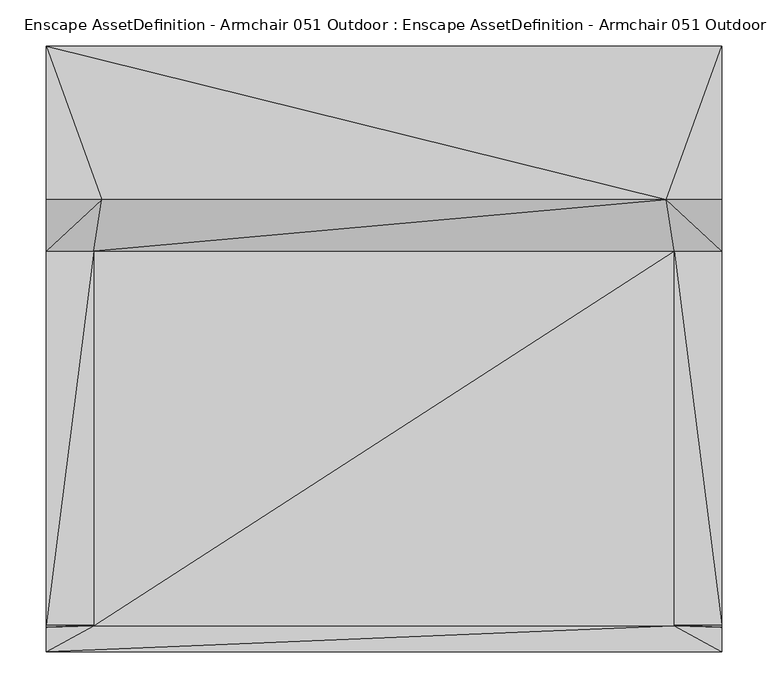
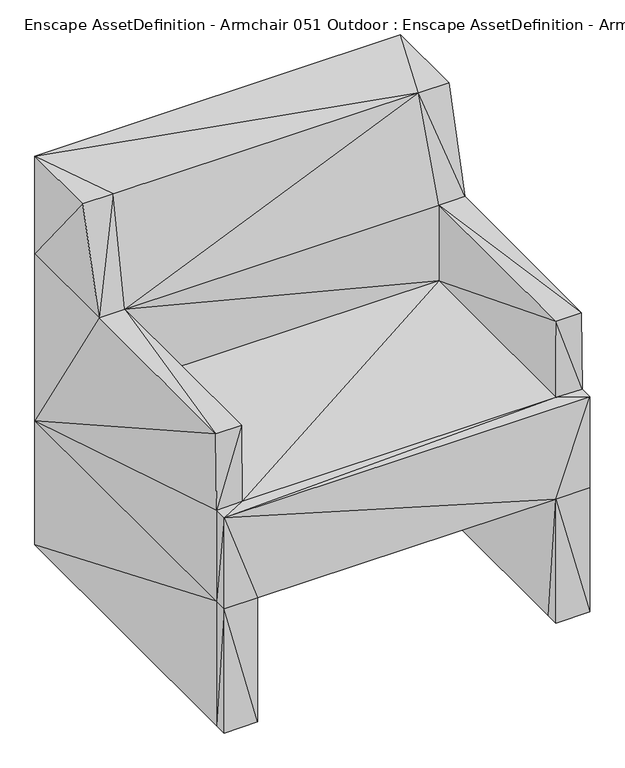
"""IFC4 building model written with IfcOpenShell, lengths in millimetres: geographic element geometry, Enscape AssetDefinition - Armchair 051 Outdoor : Enscape AssetDefinition - Armchair 051 Outdoor."""

import ifcopenshell
import ifcopenshell.guid

model = None  # the IFC model being written
_history = None  # IfcOwnerHistory: only IFC2X3 demands one
_inside = {}  # id of a spatial element -> (the spatial element, [elements in it])
_under = {}  # id of a project, library or spatial element -> (it, [spatial elements below it])
_declared = {}  # id of a project -> (the project, [libraries it declares])
_typed = {}  # id of a type object -> (the type object, [elements of that type])
_made_of = {}  # id of a material, layer set ... -> (it, [elements and type objects made of it])


def new_model(schema):
    """Start an empty IFC model of exactly this schema.

    Asked for "IFC4X3", IfcOpenShell would pick the latest addendum, in which some entities
    have other attributes; the version numbers below select the first issue.
    IFC2X3 requires an IfcOwnerHistory on every rooted entity: one is made here for all.
    """
    global model, _history
    if schema == "IFC4X3":
        model = ifcopenshell.file(schema_version=(4, 3, 0, 0))
    else:
        model = ifcopenshell.file(schema=schema)
    _inside.clear()
    _under.clear()
    _declared.clear()
    _typed.clear()
    _made_of.clear()
    _history = None
    if model.schema == "IFC2X3":
        org = make("IfcOrganization", Name="unknown")
        user = make(
            "IfcPersonAndOrganization",
            ThePerson=make("IfcPerson", FamilyName="unknown"),
            TheOrganization=org,
        )
        app = make(
            "IfcApplication",
            ApplicationDeveloper=org,
            Version="unknown",
            ApplicationFullName="unknown",
            ApplicationIdentifier="unknown",
        )
        _history = make(
            "IfcOwnerHistory",
            OwningUser=user,
            OwningApplication=app,
            ChangeAction="ADDED",
            CreationDate=0,
        )
    return model


def make(cls, **values):
    """One entity of the class cls with the attributes given. An attribute that is None is left unset."""
    return model.create_entity(
        cls, **{name: value for name, value in values.items() if value is not None}
    )


def rooted(cls, **values):
    """An entity with a GlobalId (a new one), such as an element, a storey or a relation."""
    return make(cls, GlobalId=ifcopenshell.guid.new(), OwnerHistory=_history, **values)


def si_unit(unit_type, name, prefix=None):
    """IfcSIUnit, for example si_unit("LENGTHUNIT", "METRE", prefix="MILLI")."""
    return make("IfcSIUnit", UnitType=unit_type, Prefix=prefix, Name=name)


def assignment(units):
    """IfcUnitAssignment: the units of a project."""
    return None if units is None else make("IfcUnitAssignment", Units=units)


def point(xyz):
    """IfcCartesianPoint."""
    return None if xyz is None else make("IfcCartesianPoint", Coordinates=xyz)


def direction(xyz):
    """IfcDirection."""
    return None if xyz is None else make("IfcDirection", DirectionRatios=xyz)


def frame(location, z_axis=None, x_axis=None):
    """IfcAxis2Placement3D, a coordinate frame: its origin and axes. An axis left out is left unset."""
    return make(
        "IfcAxis2Placement3D",
        Location=point(location),
        Axis=direction(z_axis),
        RefDirection=direction(x_axis),
    )


def origin():
    """The frame at (0, 0, 0) with its axes left unset."""
    return frame((0.0, 0.0, 0.0))


def place(relative_to, where):
    """IfcLocalPlacement: puts the frame where relative to a parent placement (None: the world)."""
    return make(
        "IfcLocalPlacement", PlacementRelTo=relative_to, RelativePlacement=where
    )


def context(
    kind, dimensions, precision=None, world=None, true_north=None, identifier=None
):
    """IfcGeometricRepresentationContext, for example the 3D "Model" context."""
    return make(
        "IfcGeometricRepresentationContext",
        ContextIdentifier=identifier,
        ContextType=kind,
        CoordinateSpaceDimension=dimensions,
        Precision=precision,
        WorldCoordinateSystem=world,
        TrueNorth=true_north,
    )


def project(units=None, contexts=None):
    """IfcProject with its units and contexts."""
    return rooted(
        "IfcProject",
        Name="project",
        RepresentationContexts=contexts,
        UnitsInContext=assignment(units),
    )


def spatial(cls, under=None, at=None, **own):
    """A site, building, storey or space (cls), placed at a placement, below another one or the project."""
    s = rooted(cls, ObjectPlacement=at, **own)
    if under is not None:
        _under.setdefault(under.id(), (under, []))[1].append(s)
    return s


def faces_of(points, faces, orient=None, outer=None):
    """IfcFace entities. A face is a list of loops; a loop is a list of indices into points, from 0.

    orient and outer hold one flag for each loop. By default every Orientation is true, the
    first loop of a face is its IfcFaceOuterBound and the others are IfcFaceBound.
    """
    made = []
    for i, loops in enumerate(faces):
        bounds = []
        for j, loop in enumerate(loops):
            is_outer = j == 0 if outer is None else outer[i][j]
            bounds.append(
                make(
                    "IfcFaceOuterBound" if is_outer else "IfcFaceBound",
                    Bound=make("IfcPolyLoop", Polygon=[points[k] for k in loop]),
                    Orientation=True if orient is None else orient[i][j],
                )
            )
        made.append(make("IfcFace", Bounds=bounds))
    return made


def faceted_brep(points, faces, orient=None, outer=None, voids=None):
    """IfcFacetedBrep: a solid bounded by flat faces; with voids (closed shells), ...WithVoids."""
    shared = [point(p) for p in points]
    hull = make("IfcClosedShell", CfsFaces=faces_of(shared, faces, orient, outer))
    if voids is None:
        return make("IfcFacetedBrep", Outer=hull)
    return make(
        "IfcFacetedBrepWithVoids",
        Outer=hull,
        Voids=[
            make(cls, CfsFaces=faces_of(shared, fs, o, b)) for cls, fs, o, b in voids
        ],
    )


def shape(context_of_items, identifier, shape_type, items):
    """IfcShapeRepresentation: the items that make up one representation, for example the "Body"."""
    return make(
        "IfcShapeRepresentation",
        ContextOfItems=context_of_items,
        RepresentationIdentifier=identifier,
        RepresentationType=shape_type,
        Items=items,
    )


def source(mapping_origin, context_of_items, identifier, shape_type, items):
    """IfcRepresentationMap: a shape defined once, which mapped items show again and again."""
    return make(
        "IfcRepresentationMap",
        MappingOrigin=mapping_origin,
        MappedRepresentation=shape(context_of_items, identifier, shape_type, items),
    )


def transform(
    local_origin,
    x_axis=None,
    y_axis=None,
    z_axis=None,
    scale=None,
    scale2=None,
    scale3=None,
    uniform=True,
):
    """IfcCartesianTransformationOperator3D, or its non-uniform kind. x_axis, y_axis, z_axis: its Axis1, 2, 3."""
    if uniform:
        return make(
            "IfcCartesianTransformationOperator3D",
            Axis1=direction(x_axis),
            Axis2=direction(y_axis),
            LocalOrigin=point(local_origin),
            Scale=scale,
            Axis3=direction(z_axis),
        )
    return make(
        "IfcCartesianTransformationOperator3DnonUniform",
        Axis1=direction(x_axis),
        Axis2=direction(y_axis),
        LocalOrigin=point(local_origin),
        Scale=scale,
        Axis3=direction(z_axis),
        Scale2=scale2,
        Scale3=scale3,
    )


def mapped(mapping_source, mapping_target):
    """IfcMappedItem: shows the shape of a source again, moved by a transform."""
    return make(
        "IfcMappedItem", MappingSource=mapping_source, MappingTarget=mapping_target
    )


def made_of(thing, what):
    """Note that an element or type object is made of a material, layer set ...; save() writes the relation."""
    if what is not None:
        _made_of.setdefault(what.id(), (what, []))[1].append(thing)
    return thing


def element(
    cls,
    number,
    at=None,
    inside=None,
    cuts=None,
    type_object=None,
    material=None,
    context=None,
    identifier="Body",
    shape_type=None,
    held_by="IfcProductDefinitionShape",
    body=None,
    shapes=None,
    **own,
):
    """One element of the class cls, such as IfcWall. Its Tag is "e" and its number.

    at: its placement. inside: the storey or other place that contains it. cuts: it is an
    opening in that element (IfcRelVoidsElement). A single representation is given by context,
    identifier, shape_type and body (its items); several are given by shapes. held_by: the class
    of the entity that holds the representations. save() writes the other relations.
    """
    e = rooted(cls, Tag="e%d" % number, ObjectPlacement=at, **own)
    if body is not None:
        shapes = [shape(context, identifier, shape_type, body)]
    if shapes is not None:
        e.Representation = make(held_by, Representations=shapes)
    if inside is not None:
        _inside.setdefault(inside.id(), (inside, []))[1].append(e)
    if cuts is not None:
        rooted(
            "IfcRelVoidsElement", RelatingBuildingElement=cuts, RelatedOpeningElement=e
        )
    if type_object is not None:
        _typed.setdefault(type_object.id(), (type_object, []))[1].append(e)
    return made_of(e, material)


def aggregate(whole, parts):
    """IfcRelAggregates: a whole, such as a stair, and the parts it consists of."""
    return rooted("IfcRelAggregates", RelatingObject=whole, RelatedObjects=parts)


def save(model, path):
    """Write the relations noted so far, then the file.

    IfcRelAggregates (storeys below a building ...), IfcRelContainedInSpatialStructure (elements
    in a storey), IfcRelDefinesByType, IfcRelAssociatesMaterial and IfcRelDeclares: one each for
    every whole, place, type object, material and project.
    """
    for whole, parts in _under.values():
        aggregate(whole, parts)
    for where, things in _inside.values():
        rooted(
            "IfcRelContainedInSpatialStructure",
            RelatedElements=things,
            RelatingStructure=where,
        )
    for kind, things in _typed.values():
        rooted("IfcRelDefinesByType", RelatedObjects=things, RelatingType=kind)
    for what, things in _made_of.values():
        rooted("IfcRelAssociatesMaterial", RelatedObjects=things, RelatingMaterial=what)
    for by, libraries in _declared.values():
        rooted("IfcRelDeclares", RelatingContext=by, RelatedDefinitions=libraries)
    model.write(path)


def enscape_assetdefinition_armchair_051_outdoor_enscape_3bb1fc3b(model_context):
    return source(origin(), model_context, "Body", "Brep", [
        faceted_brep([(366.5315211, -338.9842808, 262.8994286), (366.5315211, -338.9842808, 0.0), (366.5315211, -312.5311434, 0.0), (297.9772687, -338.9842808, 262.8994286), (297.9772687, -338.9842808, 0.0), (366.5315211, -312.5311732, 262.8994286), (366.5315211, 318.3681071, 0.0), (297.9772687, -312.5311434, 0.0), (366.5315211, -312.5311434, 455.7757676), (366.5315211, -338.9842808, 455.7757676), (366.5315211, 318.2037771, 262.8994286), (297.9772687, 318.3681071, 0.0), (297.9772687, 318.3681071, 262.8994286), (366.5315211, 95.6787542, 616.045773), (366.5315211, 318.3681071, 616.045773), (-299.4500101, -338.9842808, 262.8994286), (-299.4500101, 318.3681369, 262.8994286), (366.5315211, 151.5535414, 823.101759), (366.5315211, 318.3681071, 823.101759), (-366.5315211, 318.3681071, 616.045773), (306.0434759, 151.5535414, 823.101759), (-366.5315211, 318.3681071, 823.101759), (-366.5315211, 318.2038069, 262.8994286), (-366.5315211, 95.6787542, 616.045773), (-366.5315211, 151.5535414, 823.101759), (-306.0434759, 151.5535414, 823.101759), (314.7111535, 95.6787691, 616.045773), (-314.7111535, 95.6787691, 616.045773), (-366.5315211, -309.6081913, 616.045773), (-314.7111535, 95.6787542, 456.248343), (314.7111535, 95.6787542, 456.248343), (-314.7111535, -309.6081913, 616.045773), (314.7111535, -309.6081913, 616.045773), (366.5315211, -309.6081913, 616.045773), (314.6753907, -311.0696673, 456.0120404), (-314.6753907, -311.0696673, 456.0120404), (-366.5315211, -312.5311434, 455.7757676), (-366.5315211, -338.9842808, 455.7757676), (-366.5315211, -312.5311732, 262.8994286), (-366.5315211, -338.9842808, 262.8994286), (-366.5315211, 318.3681071, 0.0), (-366.5315211, -312.5311434, 0.0), (-366.5315211, -338.9842808, 0.0), (-299.4500101, -338.9842808, 0.0), (-299.4500101, -312.5311732, 0.0), (-299.4500101, 318.3681071, 0.0)], [[[0, 1, 2]], [[3, 4, 1]], [[4, 2, 1]], [[3, 1, 0]], [[5, 2, 6]], [[4, 7, 2]], [[0, 2, 5]], [[7, 6, 2]], [[0, 5, 8]], [[3, 0, 9]], [[0, 8, 9]], [[5, 10, 8]], [[5, 6, 10]], [[7, 11, 6]], [[10, 6, 11]], [[3, 7, 4]], [[3, 11, 7]], [[12, 11, 3]], [[10, 11, 12]], [[8, 10, 13]], [[13, 10, 14]], [[10, 12, 14]], [[12, 3, 15]], [[14, 12, 16]], [[12, 15, 16]], [[13, 14, 17]], [[17, 14, 18]], [[19, 18, 14]], [[14, 16, 19]], [[20, 17, 18]], [[20, 13, 17]], [[21, 18, 19]], [[18, 21, 20]], [[19, 22, 23]], [[21, 19, 24]], [[16, 22, 19]], [[24, 19, 23]], [[21, 24, 25]], [[20, 21, 25]], [[26, 13, 20]], [[25, 27, 20]], [[20, 27, 26]], [[24, 23, 25]], [[25, 23, 27]], [[23, 28, 27]], [[22, 28, 23]], [[29, 30, 27]], [[27, 31, 29]], [[27, 30, 26]], [[27, 28, 31]], [[32, 33, 26]], [[26, 33, 13]], [[30, 32, 26]], [[8, 13, 33]], [[32, 8, 33]], [[34, 8, 32]], [[34, 32, 30]], [[29, 35, 30]], [[30, 35, 34]], [[29, 31, 35]], [[28, 36, 31]], [[31, 36, 35]], [[22, 36, 28]], [[35, 36, 37]], [[22, 38, 36]], [[38, 37, 36]], [[35, 37, 34]], [[9, 8, 34]], [[34, 37, 9]], [[38, 39, 37]], [[15, 37, 39]], [[3, 37, 15]], [[3, 9, 37]], [[40, 41, 38]], [[41, 39, 38]], [[40, 38, 22]], [[41, 42, 39]], [[43, 15, 39]], [[43, 39, 42]], [[43, 16, 15]], [[44, 43, 42]], [[44, 16, 43]], [[44, 42, 41]], [[45, 44, 41]], [[45, 41, 40]], [[45, 40, 22]], [[45, 16, 44]], [[45, 22, 16]]]),
    ])


if __name__ == "__main__":
    model = new_model("IFC4")
    model_context = context("Model", 3, world=origin())
    ifc_project = project(units=[si_unit("LENGTHUNIT", "METRE", prefix="MILLI")], contexts=[model_context])
    site = spatial("IfcSite", under=ifc_project)
    building = spatial("IfcBuilding", under=site)
    placement = place(None, origin())
    enscape_assetdefinition_armchair_051_outdoor_enscape_shape = enscape_assetdefinition_armchair_051_outdoor_enscape_3bb1fc3b(model_context)
    element("IfcGeographicElement", 1, ObjectType="Enscape AssetDefinition - Armchair 051 Outdoor : Enscape AssetDefinition - Armchair 051 Outdoor", at=placement, inside=building, context=model_context, shape_type="MappedRepresentation", body=[
        mapped(enscape_assetdefinition_armchair_051_outdoor_enscape_shape, transform((0.0, 0.0, 0.0), x_axis=(1.0, 0.0, 0.0), y_axis=(0.0, 1.0, 0.0), z_axis=(0.0, 0.0, 1.0))),
    ])
    save(model, "model.ifc")

# Revit data of these elements
# Type "Enscape AssetDefinition - Armchair 051 Outdoor : Enscape AssetDefinition - Armchair 051 Outdoor"
#   EnscapeAssetSource = "REMOTE"
#   EnscapeAssetId = "e77b8969-5191-44e8-81fd-99cd1dc6d434"
#   Height = 823.102 mm
#   EnscapeNativeAssetHeight = 823.102 mm
#   Default Elevation = 0
